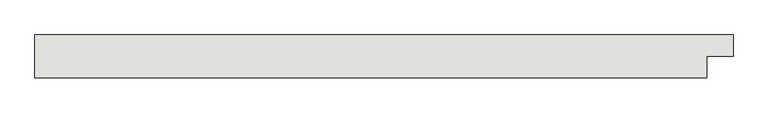
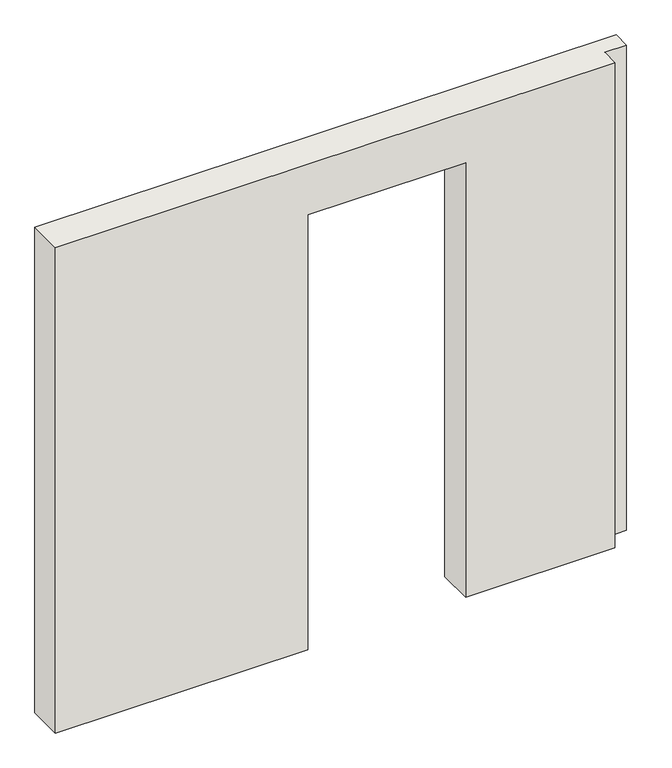
"""IFC4 building model written with IfcOpenShell, lengths in millimetres: wall geometry, 0_3d."""

import ifcopenshell
import ifcopenshell.guid

model = None  # the IFC model being written
_history = None  # IfcOwnerHistory: only IFC2X3 demands one
_inside = {}  # id of a spatial element -> (the spatial element, [elements in it])
_under = {}  # id of a project, library or spatial element -> (it, [spatial elements below it])
_declared = {}  # id of a project -> (the project, [libraries it declares])
_typed = {}  # id of a type object -> (the type object, [elements of that type])
_made_of = {}  # id of a material, layer set ... -> (it, [elements and type objects made of it])


def new_model(schema):
    """Start an empty IFC model of exactly this schema.

    Asked for "IFC4X3", IfcOpenShell would pick the latest addendum, in which some entities
    have other attributes; the version numbers below select the first issue.
    IFC2X3 requires an IfcOwnerHistory on every rooted entity: one is made here for all.
    """
    global model, _history
    if schema == "IFC4X3":
        model = ifcopenshell.file(schema_version=(4, 3, 0, 0))
    else:
        model = ifcopenshell.file(schema=schema)
    _inside.clear()
    _under.clear()
    _declared.clear()
    _typed.clear()
    _made_of.clear()
    _history = None
    if model.schema == "IFC2X3":
        org = make("IfcOrganization", Name="unknown")
        user = make(
            "IfcPersonAndOrganization",
            ThePerson=make("IfcPerson", FamilyName="unknown"),
            TheOrganization=org,
        )
        app = make(
            "IfcApplication",
            ApplicationDeveloper=org,
            Version="unknown",
            ApplicationFullName="unknown",
            ApplicationIdentifier="unknown",
        )
        _history = make(
            "IfcOwnerHistory",
            OwningUser=user,
            OwningApplication=app,
            ChangeAction="ADDED",
            CreationDate=0,
        )
    return model


def make(cls, **values):
    """One entity of the class cls with the attributes given. An attribute that is None is left unset."""
    return model.create_entity(
        cls, **{name: value for name, value in values.items() if value is not None}
    )


def rooted(cls, **values):
    """An entity with a GlobalId (a new one), such as an element, a storey or a relation."""
    return make(cls, GlobalId=ifcopenshell.guid.new(), OwnerHistory=_history, **values)


def si_unit(unit_type, name, prefix=None):
    """IfcSIUnit, for example si_unit("LENGTHUNIT", "METRE", prefix="MILLI")."""
    return make("IfcSIUnit", UnitType=unit_type, Prefix=prefix, Name=name)


def assignment(units):
    """IfcUnitAssignment: the units of a project."""
    return None if units is None else make("IfcUnitAssignment", Units=units)


def point(xyz):
    """IfcCartesianPoint."""
    return None if xyz is None else make("IfcCartesianPoint", Coordinates=xyz)


def direction(xyz):
    """IfcDirection."""
    return None if xyz is None else make("IfcDirection", DirectionRatios=xyz)


def frame(location, z_axis=None, x_axis=None):
    """IfcAxis2Placement3D, a coordinate frame: its origin and axes. An axis left out is left unset."""
    return make(
        "IfcAxis2Placement3D",
        Location=point(location),
        Axis=direction(z_axis),
        RefDirection=direction(x_axis),
    )


def origin():
    """The frame at (0, 0, 0) with its axes left unset."""
    return frame((0.0, 0.0, 0.0))


def place(relative_to, where):
    """IfcLocalPlacement: puts the frame where relative to a parent placement (None: the world)."""
    return make(
        "IfcLocalPlacement", PlacementRelTo=relative_to, RelativePlacement=where
    )


def context(
    kind, dimensions, precision=None, world=None, true_north=None, identifier=None
):
    """IfcGeometricRepresentationContext, for example the 3D "Model" context."""
    return make(
        "IfcGeometricRepresentationContext",
        ContextIdentifier=identifier,
        ContextType=kind,
        CoordinateSpaceDimension=dimensions,
        Precision=precision,
        WorldCoordinateSystem=world,
        TrueNorth=true_north,
    )


def project(units=None, contexts=None):
    """IfcProject with its units and contexts."""
    return rooted(
        "IfcProject",
        Name="project",
        RepresentationContexts=contexts,
        UnitsInContext=assignment(units),
    )


def spatial(cls, under=None, at=None, **own):
    """A site, building, storey or space (cls), placed at a placement, below another one or the project."""
    s = rooted(cls, ObjectPlacement=at, **own)
    if under is not None:
        _under.setdefault(under.id(), (under, []))[1].append(s)
    return s


def faces_of(points, faces, orient=None, outer=None):
    """IfcFace entities. A face is a list of loops; a loop is a list of indices into points, from 0.

    orient and outer hold one flag for each loop. By default every Orientation is true, the
    first loop of a face is its IfcFaceOuterBound and the others are IfcFaceBound.
    """
    made = []
    for i, loops in enumerate(faces):
        bounds = []
        for j, loop in enumerate(loops):
            is_outer = j == 0 if outer is None else outer[i][j]
            bounds.append(
                make(
                    "IfcFaceOuterBound" if is_outer else "IfcFaceBound",
                    Bound=make("IfcPolyLoop", Polygon=[points[k] for k in loop]),
                    Orientation=True if orient is None else orient[i][j],
                )
            )
        made.append(make("IfcFace", Bounds=bounds))
    return made


def faceted_brep(points, faces, orient=None, outer=None, voids=None):
    """IfcFacetedBrep: a solid bounded by flat faces; with voids (closed shells), ...WithVoids."""
    shared = [point(p) for p in points]
    hull = make("IfcClosedShell", CfsFaces=faces_of(shared, faces, orient, outer))
    if voids is None:
        return make("IfcFacetedBrep", Outer=hull)
    return make(
        "IfcFacetedBrepWithVoids",
        Outer=hull,
        Voids=[
            make(cls, CfsFaces=faces_of(shared, fs, o, b)) for cls, fs, o, b in voids
        ],
    )


def shape(context_of_items, identifier, shape_type, items):
    """IfcShapeRepresentation: the items that make up one representation, for example the "Body"."""
    return make(
        "IfcShapeRepresentation",
        ContextOfItems=context_of_items,
        RepresentationIdentifier=identifier,
        RepresentationType=shape_type,
        Items=items,
    )


def source(mapping_origin, context_of_items, identifier, shape_type, items):
    """IfcRepresentationMap: a shape defined once, which mapped items show again and again."""
    return make(
        "IfcRepresentationMap",
        MappingOrigin=mapping_origin,
        MappedRepresentation=shape(context_of_items, identifier, shape_type, items),
    )


def transform(
    local_origin,
    x_axis=None,
    y_axis=None,
    z_axis=None,
    scale=None,
    scale2=None,
    scale3=None,
    uniform=True,
):
    """IfcCartesianTransformationOperator3D, or its non-uniform kind. x_axis, y_axis, z_axis: its Axis1, 2, 3."""
    if uniform:
        return make(
            "IfcCartesianTransformationOperator3D",
            Axis1=direction(x_axis),
            Axis2=direction(y_axis),
            LocalOrigin=point(local_origin),
            Scale=scale,
            Axis3=direction(z_axis),
        )
    return make(
        "IfcCartesianTransformationOperator3DnonUniform",
        Axis1=direction(x_axis),
        Axis2=direction(y_axis),
        LocalOrigin=point(local_origin),
        Scale=scale,
        Axis3=direction(z_axis),
        Scale2=scale2,
        Scale3=scale3,
    )


def mapped(mapping_source, mapping_target):
    """IfcMappedItem: shows the shape of a source again, moved by a transform."""
    return make(
        "IfcMappedItem", MappingSource=mapping_source, MappingTarget=mapping_target
    )


def made_of(thing, what):
    """Note that an element or type object is made of a material, layer set ...; save() writes the relation."""
    if what is not None:
        _made_of.setdefault(what.id(), (what, []))[1].append(thing)
    return thing


def element(
    cls,
    number,
    at=None,
    inside=None,
    cuts=None,
    type_object=None,
    material=None,
    context=None,
    identifier="Body",
    shape_type=None,
    held_by="IfcProductDefinitionShape",
    body=None,
    shapes=None,
    **own,
):
    """One element of the class cls, such as IfcWall. Its Tag is "e" and its number.

    at: its placement. inside: the storey or other place that contains it. cuts: it is an
    opening in that element (IfcRelVoidsElement). A single representation is given by context,
    identifier, shape_type and body (its items); several are given by shapes. held_by: the class
    of the entity that holds the representations. save() writes the other relations.
    """
    e = rooted(cls, Tag="e%d" % number, ObjectPlacement=at, **own)
    if body is not None:
        shapes = [shape(context, identifier, shape_type, body)]
    if shapes is not None:
        e.Representation = make(held_by, Representations=shapes)
    if inside is not None:
        _inside.setdefault(inside.id(), (inside, []))[1].append(e)
    if cuts is not None:
        rooted(
            "IfcRelVoidsElement", RelatingBuildingElement=cuts, RelatedOpeningElement=e
        )
    if type_object is not None:
        _typed.setdefault(type_object.id(), (type_object, []))[1].append(e)
    return made_of(e, material)


def aggregate(whole, parts):
    """IfcRelAggregates: a whole, such as a stair, and the parts it consists of."""
    return rooted("IfcRelAggregates", RelatingObject=whole, RelatedObjects=parts)


def save(model, path):
    """Write the relations noted so far, then the file.

    IfcRelAggregates (storeys below a building ...), IfcRelContainedInSpatialStructure (elements
    in a storey), IfcRelDefinesByType, IfcRelAssociatesMaterial and IfcRelDeclares: one each for
    every whole, place, type object, material and project.
    """
    for whole, parts in _under.values():
        aggregate(whole, parts)
    for where, things in _inside.values():
        rooted(
            "IfcRelContainedInSpatialStructure",
            RelatedElements=things,
            RelatingStructure=where,
        )
    for kind, things in _typed.values():
        rooted("IfcRelDefinesByType", RelatedObjects=things, RelatingType=kind)
    for what, things in _made_of.values():
        rooted("IfcRelAssociatesMaterial", RelatedObjects=things, RelatingMaterial=what)
    for by, libraries in _declared.values():
        rooted("IfcRelDeclares", RelatingContext=by, RelatedDefinitions=libraries)
    model.write(path)


def wall_2d906ff1(model_context):
    return source(origin(), model_context, "Body", "Brep", [
        faceted_brep([(1416.8093021, 0.0, 0.0), (1416.8093021, 200.0, 0.0), (1416.8093021, 200.0, 2580.0), (1416.8093021, 0.0, 2580.0), (2301.8093021, 200.0, 2580.0), (2301.8093021, 0.0, 2580.0), (2301.8093021, 200.0, 0.0), (2301.8093021, 0.0, 0.0), (0.0, 200.0, 0.0), (0.0, 200.0, 2880.0), (3261.9364642, 200.0, 2880.0), (3261.9364642, 200.0, 0.0), (0.0, 0.0, 0.0), (0.0, 0.0, 2880.0), (3261.9364642, 100.0, 0.0), (3261.9364642, 100.0, 2880.0), (3139.9364642, 100.0, 0.0), (3139.9364642, 100.0, 2880.0), (3139.9364642, 0.0, 0.0), (3139.9364642, 0.0, 2880.0)], [[[0, 1, 2, 3]], [[2, 4, 5, 3]], [[6, 7, 5, 4]], [[6, 4, 2, 1, 8, 9, 10, 11]], [[1, 0, 12, 8]], [[8, 12, 13, 9]], [[14, 11, 10, 15]], [[16, 14, 15, 17]], [[18, 16, 17, 19]], [[5, 7, 18, 19, 13, 12, 0, 3]], [[13, 19, 17, 15, 10, 9]], [[7, 6, 11, 14, 16, 18]]]),
    ])


if __name__ == "__main__":
    model = new_model("IFC4")
    model_context = context("Model", 3, world=origin())
    ifc_project = project(units=[si_unit("LENGTHUNIT", "METRE", prefix="MILLI")], contexts=[model_context])
    site = spatial("IfcSite", under=ifc_project)
    building = spatial("IfcBuilding", under=site)
    placement = place(None, origin())
    wall_shape = wall_2d906ff1(model_context)
    element("IfcWall", 1, ObjectType="0_3d", at=placement, inside=building, context=model_context, shape_type="MappedRepresentation", body=[
        mapped(wall_shape, transform((0.0, 0.0, 0.0), x_axis=(1.0, 0.0, 0.0), y_axis=(0.0, 1.0, 0.0), z_axis=(0.0, 0.0, 1.0))),
    ])
    save(model, "model.ifc")

# Revit data of these elements
# Element 1 (IfcWall, "0_3d")
#   Materials on its faces: "material wardrobe b 1"
# Materials
#   "material wardrobe b 1": class "Unassigned", colour RGB 128 128 128, transparency 0
